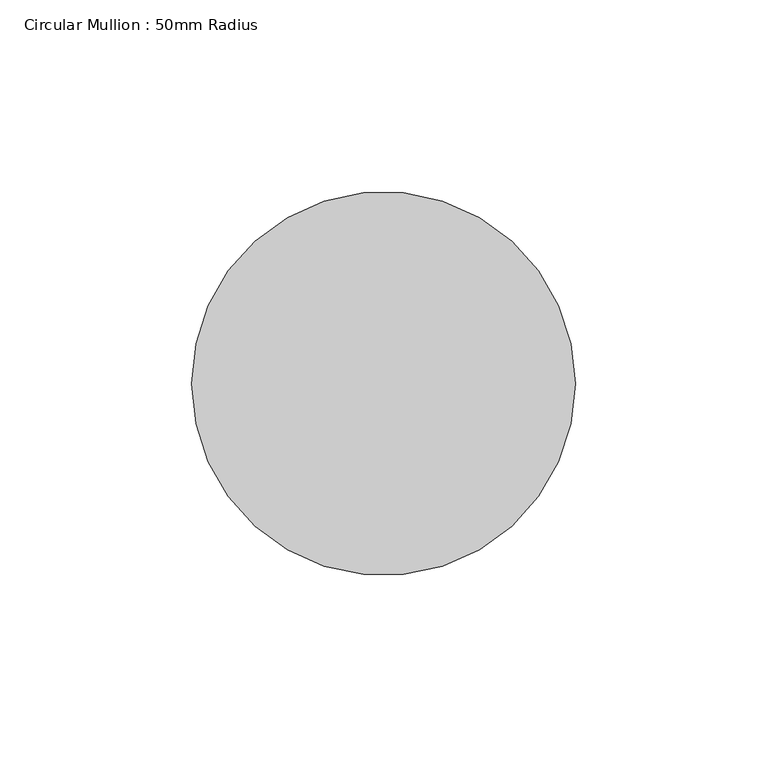
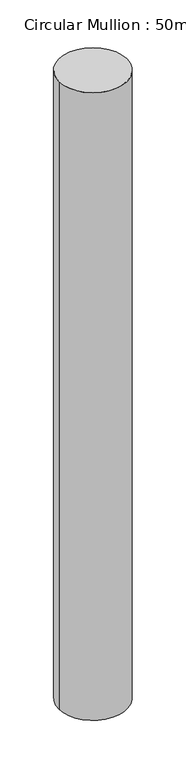
"""IFC4 building model written with IfcOpenShell, lengths in millimetres: member geometry, Circular Mullion : 50mm Radius."""

from ifc_helpers import new_model, si_unit, point, frame, origin, origin_2d, place, context, project, spatial, circle_curve, trimmed, segment, composite_curve, outline, extrude, source, transform, mapped, element, save


def circular_mullion_50mm_radius_0269846c(model_context):
    return source(origin(), model_context, "Body", "SweptSolid", [
        extrude(outline(composite_curve([segment(trimmed(circle_curve(origin_2d(), 50.0), [point((50.0, 0.0))], [point((-50.0, 0.0))], False, "CARTESIAN"), True, "CONTINUOUS"), segment(trimmed(circle_curve(origin_2d(), 50.0), [point((-50.0, 0.0))], [point((50.0, 0.0))], False, "CARTESIAN"), True, "CONTINUOUS")], self_intersect=False)), frame((0.0, 0.0, -972.9044034), z_axis=(0.0, 0.0, 1.0), x_axis=(1.0, 0.0, 0.0)), (0.0, 0.0, 1.0), 972.9044034),
    ])


if __name__ == "__main__":
    model = new_model("IFC4")
    model_context = context("Model", 3, world=origin())
    ifc_project = project(units=[si_unit("LENGTHUNIT", "METRE", prefix="MILLI")], contexts=[model_context])
    site = spatial("IfcSite", under=ifc_project)
    building = spatial("IfcBuilding", under=site)
    placement = place(None, origin())
    circular_mullion_50mm_radius_shape = circular_mullion_50mm_radius_0269846c(model_context)
    element("IfcMember", 1, ObjectType="Circular Mullion : 50mm Radius", at=placement, inside=building, context=model_context, shape_type="MappedRepresentation", body=[
        mapped(circular_mullion_50mm_radius_shape, transform((0.0, 0.0, 0.0), x_axis=(1.0, 0.0, 0.0), y_axis=(0.0, 1.0, 0.0), z_axis=(0.0, 0.0, 1.0))),
    ])
    save(model, "model.ifc")

# Revit data of these elements
# Type "Circular Mullion : 50mm Radius"
#   built-in parameter 1007350 = 0.164042 (stored number, unit not read)
# Element 1 (IfcMember, "Circular Mullion : 50mm Radius")
#   Materials on its faces: "Aluminium"
# Materials
#   "Aluminium": class "Metal", colour RGB 247 247 247, transparency 0, Description = "Aluminium 6061", Cost = 0
